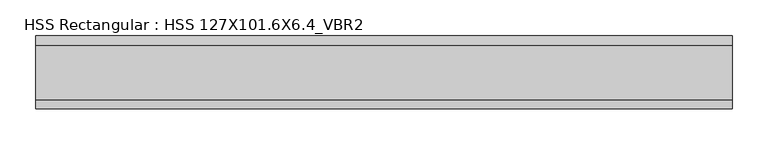
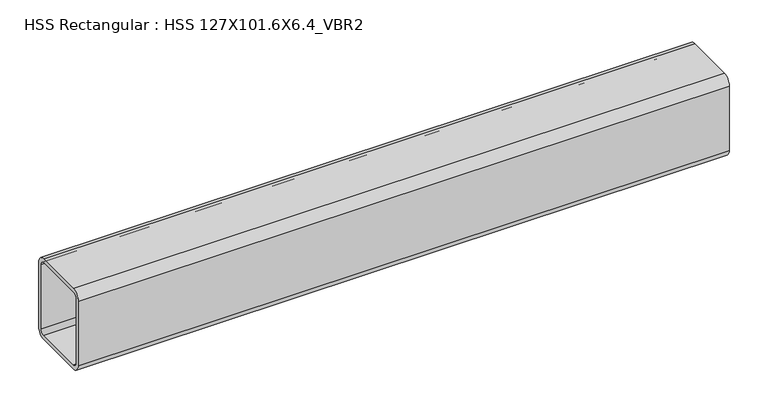
"""IFC4 building model written with IfcOpenShell, lengths in millimetres: member geometry, HSS Rectangular : HSS 127X101.6X6.4_VBR2."""

from ifc_helpers import new_model, si_unit, point, frame, frame_2d, origin, place, context, project, spatial, polyline, circle_curve, trimmed, segment, composite_curve, outline, extrude, source, transform, mapped, element, save


def hss_rectangular_hss_127x101_6x6_4_vbr2_a0ef1968(model_context):
    return source(origin(), model_context, "Body", "SweptSolid", [
        extrude(outline(composite_curve([segment(polyline([(50.8, 50.8), (50.8, -50.8)]), True, "CONTINUOUS"), segment(trimmed(circle_curve(frame_2d((38.1, -50.8)), 12.7), [point((50.8, -50.8))], [point((38.1, -63.5))], False, "CARTESIAN"), True, "CONTINUOUS"), segment(polyline([(38.1, -63.5), (-38.1, -63.5)]), True, "CONTINUOUS"), segment(trimmed(circle_curve(frame_2d((-38.1, -50.8)), 12.7), [point((-38.1, -63.5))], [point((-50.8, -50.8))], False, "CARTESIAN"), True, "CONTINUOUS"), segment(polyline([(-50.8, -50.8), (-50.8, 50.8)]), True, "CONTINUOUS"), segment(trimmed(circle_curve(frame_2d((-38.1, 50.8)), 12.7), [point((-50.8, 50.8))], [point((-38.1, 63.5))], False, "CARTESIAN"), True, "CONTINUOUS"), segment(polyline([(-38.1, 63.5), (38.1, 63.5)]), True, "CONTINUOUS"), segment(trimmed(circle_curve(frame_2d((38.1, 50.8)), 12.7), [point((38.1, 63.5))], [point((50.8, 50.8))], False, "CARTESIAN"), True, "CONTINUOUS")], self_intersect=False), holes=[composite_curve([segment(trimmed(circle_curve(frame_2d((-38.1, 50.8)), 6.35), [point((-38.1, 57.15))], [point((-44.45, 50.8))], True, "CARTESIAN"), True, "CONTINUOUS"), segment(polyline([(-44.45, 50.8), (-44.45, -50.8)]), True, "CONTINUOUS"), segment(trimmed(circle_curve(frame_2d((-38.1, -50.8)), 6.35), [point((-44.45, -50.8))], [point((-38.1, -57.15))], True, "CARTESIAN"), True, "CONTINUOUS"), segment(polyline([(-38.1, -57.15), (38.1, -57.15)]), True, "CONTINUOUS"), segment(trimmed(circle_curve(frame_2d((38.1, -50.8)), 6.35), [point((38.1, -57.15))], [point((44.45, -50.8))], True, "CARTESIAN"), True, "CONTINUOUS"), segment(polyline([(44.45, -50.8), (44.45, 50.8)]), True, "CONTINUOUS"), segment(trimmed(circle_curve(frame_2d((38.1, 50.8)), 6.35), [point((44.45, 50.8))], [point((38.1, 57.15))], True, "CARTESIAN"), True, "CONTINUOUS"), segment(polyline([(38.1, 57.15), (-38.1, 57.15)]), True, "CONTINUOUS")], self_intersect=False)]), frame((-539.729906, 0.0, 0.0), z_axis=(1.0, 0.0, 0.0), x_axis=(0.0, 1.0, 0.0)), (0.0, 0.0, 1.0), 969.0422579),
    ])


if __name__ == "__main__":
    model = new_model("IFC4")
    model_context = context("Model", 3, world=origin())
    ifc_project = project(units=[si_unit("LENGTHUNIT", "METRE", prefix="MILLI")], contexts=[model_context])
    site = spatial("IfcSite", under=ifc_project)
    building = spatial("IfcBuilding", under=site)
    placement = place(None, origin())
    hss_rectangular_hss_127x101_6x6_4_vbr2_shape = hss_rectangular_hss_127x101_6x6_4_vbr2_a0ef1968(model_context)
    element("IfcMember", 1, ObjectType="HSS Rectangular : HSS 127X101.6X6.4_VBR2", at=placement, inside=building, context=model_context, shape_type="MappedRepresentation", body=[
        mapped(hss_rectangular_hss_127x101_6x6_4_vbr2_shape, transform((0.0, 0.0, 0.0), x_axis=(1.0, 0.0, 0.0), y_axis=(0.0, 1.0, 0.0), z_axis=(0.0, 0.0, 1.0))),
    ])
    save(model, "model.ifc")

# Revit data of these elements
# Type "HSS Rectangular : HSS 127X101.6X6.4_VBR2"
#   Section Name Key = "HSS5X4X1/4"
#   Assembly Code = "B10"
#   Width = 10.16 cm
#   Wall Nominal Thickness = 0.635 cm
#   Wall Design Thickness = 0.5918 cm
#   Torsional Moment of Inertia = 749.217 cm⁴
#   Torsional Modulus = 136.34 cm³
#   Section Area = 24.7741 cm²
#   Plastic Modulus weak axis = 91.2759 cm³
#   Plastic Modulus strong axis = 106.352 cm³
#   Perimeter = 0.435254 m²/m
#   Outer Fillet = 1.27 cm
#   Nominal Weight = 20.7004 kgf/m
#   Moment of Inertia weak axis = 393.755 cm⁴
#   Moment of Inertia strong axis = 557.75 cm⁴
#   Inner Fillet = 0.635 cm
#   Height = 12.7 cm
#   Elastic Modulus weak axis = 77.5108 cm³
#   Elastic Modulus strong axis = 87.6708 cm³
#   Centroid Vertical = 6.35 cm
#   Centroid Horizontal = 5.08 cm
#   Length [instance default] = 1524 mm
#   Structural Material [instance default] = Steel ASTM A500, Grade C, Rectangular and Square
#   Principal Axes Angle = 0
# Element 1 (IfcMember, "HSS Rectangular : HSS 127X101.6X6.4_VBR2")
#   Materials on its faces: "Steel ASTM A500, Grade C, Rectangular and Square"
# Materials
#   "Steel ASTM A500, Grade C, Rectangular and Square": class "Metal", colour RGB 120 120 120, transparency 0, Description = "Carbon steel", Cost = 0
